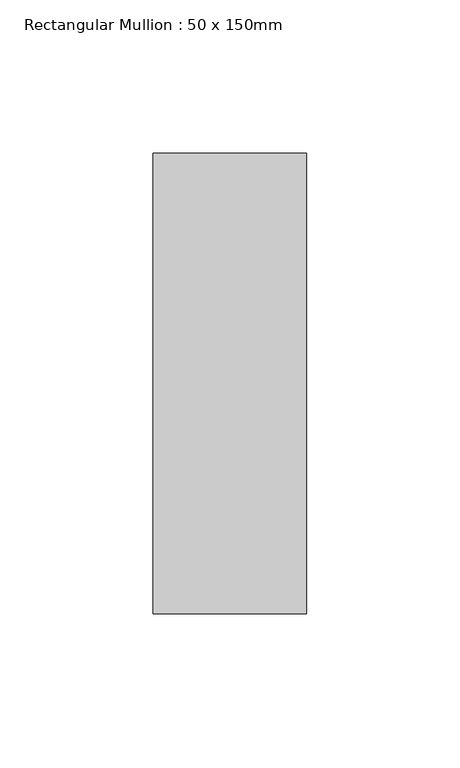
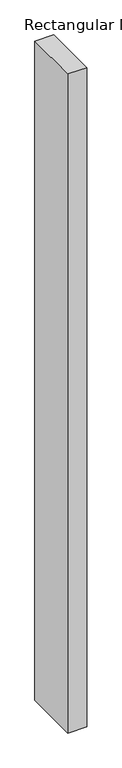
"""IFC4 building model written with IfcOpenShell, lengths in millimetres: member geometry, Rectangular Mullion : 50 x 150mm."""

from ifc_helpers import new_model, si_unit, frame, origin, place, context, project, spatial, polyline, outline, extrude, source, transform, mapped, element, save


def rectangular_mullion_50_x_150mm_4a09804a(model_context):
    return source(origin(), model_context, "Body", "SweptSolid", [
        extrude(outline(polyline([(25.0, 75.0), (25.0, -75.0), (-25.0, -75.0), (-25.0, 75.0), (25.0, 75.0)])), frame((0.0, 0.0, -1838.8888888), z_axis=(0.0, 0.0, 1.0), x_axis=(1.0, 0.0, 0.0)), (0.0, 0.0, 1.0), 1838.8888888),
    ])


if __name__ == "__main__":
    model = new_model("IFC4")
    model_context = context("Model", 3, world=origin())
    ifc_project = project(units=[si_unit("LENGTHUNIT", "METRE", prefix="MILLI")], contexts=[model_context])
    site = spatial("IfcSite", under=ifc_project)
    building = spatial("IfcBuilding", under=site)
    placement = place(None, origin())
    rectangular_mullion_50_x_150mm_shape = rectangular_mullion_50_x_150mm_4a09804a(model_context)
    element("IfcMember", 1, ObjectType="Rectangular Mullion : 50 x 150mm", at=placement, inside=building, context=model_context, shape_type="MappedRepresentation", body=[
        mapped(rectangular_mullion_50_x_150mm_shape, transform((0.0, 0.0, 0.0), x_axis=(1.0, 0.0, 0.0), y_axis=(0.0, 1.0, 0.0), z_axis=(0.0, 0.0, 1.0))),
    ])
    save(model, "model.ifc")

# Revit data of these elements
# Type "Rectangular Mullion : 50 x 150mm"
#   built-in parameter 1007304 = 0.492126 (stored number, unit not read)
#   built-in parameter 1007301 = 0.082021 (stored number, unit not read)
#   built-in parameter 1007300 = 0.082021 (stored number, unit not read)
# Element 1 (IfcMember, "Rectangular Mullion : 50 x 150mm")
#   Materials on its faces: "Metal - Aluminium"
# Materials
#   "Metal - Aluminium": class "Metal", colour RGB 247 247 247, transparency 0
